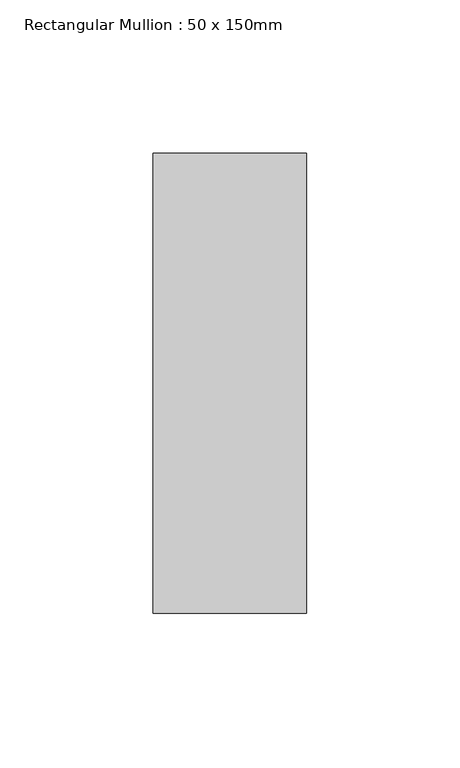
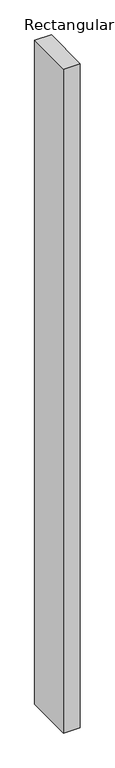
"""IFC4 building model written with IfcOpenShell, lengths in millimetres: member geometry, Rectangular Mullion : 50 x 150mm."""

from ifc_helpers import new_model, si_unit, frame, origin, place, context, project, spatial, polyline, outline, extrude, source, transform, mapped, element, save


def rectangular_mullion_50_x_150mm_2d9f00d1(model_context):
    return source(origin(), model_context, "Body", "SweptSolid", [
        extrude(outline(polyline([(25.0, 75.0), (25.0, -75.0), (-25.0, -75.0), (-25.0, 75.0), (25.0, 75.0)])), frame((0.0, 0.0, -2105.4462072), z_axis=(0.0, 0.0, 1.0), x_axis=(1.0, 0.0, 0.0)), (0.0, 0.0, 1.0), 2105.4462072),
    ])


if __name__ == "__main__":
    model = new_model("IFC4")
    model_context = context("Model", 3, world=origin())
    ifc_project = project(units=[si_unit("LENGTHUNIT", "METRE", prefix="MILLI")], contexts=[model_context])
    site = spatial("IfcSite", under=ifc_project)
    building = spatial("IfcBuilding", under=site)
    placement = place(None, origin())
    rectangular_mullion_50_x_150mm_shape = rectangular_mullion_50_x_150mm_2d9f00d1(model_context)
    element("IfcMember", 1, ObjectType="Rectangular Mullion : 50 x 150mm", at=placement, inside=building, context=model_context, shape_type="MappedRepresentation", body=[
        mapped(rectangular_mullion_50_x_150mm_shape, transform((0.0, 0.0, 0.0), x_axis=(1.0, 0.0, 0.0), y_axis=(0.0, 1.0, 0.0), z_axis=(0.0, 0.0, 1.0))),
    ])
    save(model, "model.ifc")

# Revit data of these elements
# Type "Rectangular Mullion : 50 x 150mm"
#   built-in parameter 1007304 = 0.492126 (stored number, unit not read)
#   built-in parameter 1007301 = 0.082021 (stored number, unit not read)
#   built-in parameter 1007300 = 0.082021 (stored number, unit not read)
# Element 1 (IfcMember, "Rectangular Mullion : 50 x 150mm")
#   Materials on its faces: "Aluminium"
# Materials
#   "Aluminium": class "Metal", colour RGB 247 247 247, transparency 0, Description = "Aluminium 6061", Cost = 0
